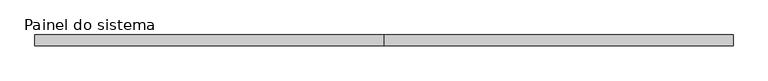
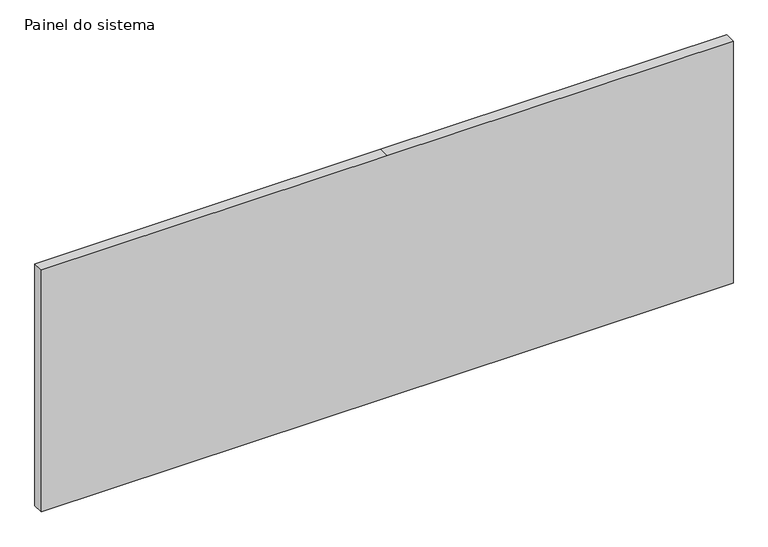
"""IFC4 building model written with IfcOpenShell, lengths in millimetres: plate geometry, Painel do sistema : Envidraçado."""

import ifcopenshell
import ifcopenshell.guid

model = None  # the IFC model being written
_history = None  # IfcOwnerHistory: only IFC2X3 demands one
_inside = {}  # id of a spatial element -> (the spatial element, [elements in it])
_under = {}  # id of a project, library or spatial element -> (it, [spatial elements below it])
_declared = {}  # id of a project -> (the project, [libraries it declares])
_typed = {}  # id of a type object -> (the type object, [elements of that type])
_made_of = {}  # id of a material, layer set ... -> (it, [elements and type objects made of it])


def new_model(schema):
    """Start an empty IFC model of exactly this schema.

    Asked for "IFC4X3", IfcOpenShell would pick the latest addendum, in which some entities
    have other attributes; the version numbers below select the first issue.
    IFC2X3 requires an IfcOwnerHistory on every rooted entity: one is made here for all.
    """
    global model, _history
    if schema == "IFC4X3":
        model = ifcopenshell.file(schema_version=(4, 3, 0, 0))
    else:
        model = ifcopenshell.file(schema=schema)
    _inside.clear()
    _under.clear()
    _declared.clear()
    _typed.clear()
    _made_of.clear()
    _history = None
    if model.schema == "IFC2X3":
        org = make("IfcOrganization", Name="unknown")
        user = make(
            "IfcPersonAndOrganization",
            ThePerson=make("IfcPerson", FamilyName="unknown"),
            TheOrganization=org,
        )
        app = make(
            "IfcApplication",
            ApplicationDeveloper=org,
            Version="unknown",
            ApplicationFullName="unknown",
            ApplicationIdentifier="unknown",
        )
        _history = make(
            "IfcOwnerHistory",
            OwningUser=user,
            OwningApplication=app,
            ChangeAction="ADDED",
            CreationDate=0,
        )
    return model


def make(cls, **values):
    """One entity of the class cls with the attributes given. An attribute that is None is left unset."""
    return model.create_entity(
        cls, **{name: value for name, value in values.items() if value is not None}
    )


def rooted(cls, **values):
    """An entity with a GlobalId (a new one), such as an element, a storey or a relation."""
    return make(cls, GlobalId=ifcopenshell.guid.new(), OwnerHistory=_history, **values)


def si_unit(unit_type, name, prefix=None):
    """IfcSIUnit, for example si_unit("LENGTHUNIT", "METRE", prefix="MILLI")."""
    return make("IfcSIUnit", UnitType=unit_type, Prefix=prefix, Name=name)


def assignment(units):
    """IfcUnitAssignment: the units of a project."""
    return None if units is None else make("IfcUnitAssignment", Units=units)


def point(xyz):
    """IfcCartesianPoint."""
    return None if xyz is None else make("IfcCartesianPoint", Coordinates=xyz)


def direction(xyz):
    """IfcDirection."""
    return None if xyz is None else make("IfcDirection", DirectionRatios=xyz)


def frame(location, z_axis=None, x_axis=None):
    """IfcAxis2Placement3D, a coordinate frame: its origin and axes. An axis left out is left unset."""
    return make(
        "IfcAxis2Placement3D",
        Location=point(location),
        Axis=direction(z_axis),
        RefDirection=direction(x_axis),
    )


def origin():
    """The frame at (0, 0, 0) with its axes left unset."""
    return frame((0.0, 0.0, 0.0))


def place(relative_to, where):
    """IfcLocalPlacement: puts the frame where relative to a parent placement (None: the world)."""
    return make(
        "IfcLocalPlacement", PlacementRelTo=relative_to, RelativePlacement=where
    )


def context(
    kind, dimensions, precision=None, world=None, true_north=None, identifier=None
):
    """IfcGeometricRepresentationContext, for example the 3D "Model" context."""
    return make(
        "IfcGeometricRepresentationContext",
        ContextIdentifier=identifier,
        ContextType=kind,
        CoordinateSpaceDimension=dimensions,
        Precision=precision,
        WorldCoordinateSystem=world,
        TrueNorth=true_north,
    )


def project(units=None, contexts=None):
    """IfcProject with its units and contexts."""
    return rooted(
        "IfcProject",
        Name="project",
        RepresentationContexts=contexts,
        UnitsInContext=assignment(units),
    )


def spatial(cls, under=None, at=None, **own):
    """A site, building, storey or space (cls), placed at a placement, below another one or the project."""
    s = rooted(cls, ObjectPlacement=at, **own)
    if under is not None:
        _under.setdefault(under.id(), (under, []))[1].append(s)
    return s


def polyline(points):
    """IfcPolyline through the points."""
    return make("IfcPolyline", Points=[point(p) for p in points])


def outline(outer, holes=None, kind="AREA"):
    """IfcArbitraryClosedProfileDef: a profile drawn as a closed curve; with holes, ...WithVoids."""
    if holes is None:
        return make("IfcArbitraryClosedProfileDef", ProfileType=kind, OuterCurve=outer)
    return make(
        "IfcArbitraryProfileDefWithVoids",
        ProfileType=kind,
        OuterCurve=outer,
        InnerCurves=holes,
    )


def extrude(swept, where, along, depth):
    """IfcExtrudedAreaSolid: the profile swept, set in the frame where, extruded along a direction by depth."""
    return make(
        "IfcExtrudedAreaSolid",
        SweptArea=swept,
        Position=where,
        ExtrudedDirection=direction(along),
        Depth=depth,
    )


def shape(context_of_items, identifier, shape_type, items):
    """IfcShapeRepresentation: the items that make up one representation, for example the "Body"."""
    return make(
        "IfcShapeRepresentation",
        ContextOfItems=context_of_items,
        RepresentationIdentifier=identifier,
        RepresentationType=shape_type,
        Items=items,
    )


def source(mapping_origin, context_of_items, identifier, shape_type, items):
    """IfcRepresentationMap: a shape defined once, which mapped items show again and again."""
    return make(
        "IfcRepresentationMap",
        MappingOrigin=mapping_origin,
        MappedRepresentation=shape(context_of_items, identifier, shape_type, items),
    )


def transform(
    local_origin,
    x_axis=None,
    y_axis=None,
    z_axis=None,
    scale=None,
    scale2=None,
    scale3=None,
    uniform=True,
):
    """IfcCartesianTransformationOperator3D, or its non-uniform kind. x_axis, y_axis, z_axis: its Axis1, 2, 3."""
    if uniform:
        return make(
            "IfcCartesianTransformationOperator3D",
            Axis1=direction(x_axis),
            Axis2=direction(y_axis),
            LocalOrigin=point(local_origin),
            Scale=scale,
            Axis3=direction(z_axis),
        )
    return make(
        "IfcCartesianTransformationOperator3DnonUniform",
        Axis1=direction(x_axis),
        Axis2=direction(y_axis),
        LocalOrigin=point(local_origin),
        Scale=scale,
        Axis3=direction(z_axis),
        Scale2=scale2,
        Scale3=scale3,
    )


def mapped(mapping_source, mapping_target):
    """IfcMappedItem: shows the shape of a source again, moved by a transform."""
    return make(
        "IfcMappedItem", MappingSource=mapping_source, MappingTarget=mapping_target
    )


def made_of(thing, what):
    """Note that an element or type object is made of a material, layer set ...; save() writes the relation."""
    if what is not None:
        _made_of.setdefault(what.id(), (what, []))[1].append(thing)
    return thing


def element(
    cls,
    number,
    at=None,
    inside=None,
    cuts=None,
    type_object=None,
    material=None,
    context=None,
    identifier="Body",
    shape_type=None,
    held_by="IfcProductDefinitionShape",
    body=None,
    shapes=None,
    **own,
):
    """One element of the class cls, such as IfcWall. Its Tag is "e" and its number.

    at: its placement. inside: the storey or other place that contains it. cuts: it is an
    opening in that element (IfcRelVoidsElement). A single representation is given by context,
    identifier, shape_type and body (its items); several are given by shapes. held_by: the class
    of the entity that holds the representations. save() writes the other relations.
    """
    e = rooted(cls, Tag="e%d" % number, ObjectPlacement=at, **own)
    if body is not None:
        shapes = [shape(context, identifier, shape_type, body)]
    if shapes is not None:
        e.Representation = make(held_by, Representations=shapes)
    if inside is not None:
        _inside.setdefault(inside.id(), (inside, []))[1].append(e)
    if cuts is not None:
        rooted(
            "IfcRelVoidsElement", RelatingBuildingElement=cuts, RelatedOpeningElement=e
        )
    if type_object is not None:
        _typed.setdefault(type_object.id(), (type_object, []))[1].append(e)
    return made_of(e, material)


def aggregate(whole, parts):
    """IfcRelAggregates: a whole, such as a stair, and the parts it consists of."""
    return rooted("IfcRelAggregates", RelatingObject=whole, RelatedObjects=parts)


def save(model, path):
    """Write the relations noted so far, then the file.

    IfcRelAggregates (storeys below a building ...), IfcRelContainedInSpatialStructure (elements
    in a storey), IfcRelDefinesByType, IfcRelAssociatesMaterial and IfcRelDeclares: one each for
    every whole, place, type object, material and project.
    """
    for whole, parts in _under.values():
        aggregate(whole, parts)
    for where, things in _inside.values():
        rooted(
            "IfcRelContainedInSpatialStructure",
            RelatedElements=things,
            RelatingStructure=where,
        )
    for kind, things in _typed.values():
        rooted("IfcRelDefinesByType", RelatedObjects=things, RelatingType=kind)
    for what, things in _made_of.values():
        rooted("IfcRelAssociatesMaterial", RelatedObjects=things, RelatingMaterial=what)
    for by, libraries in _declared.values():
        rooted("IfcRelDeclares", RelatingContext=by, RelatedDefinitions=libraries)
    model.write(path)


def painel_do_sistema_93f97b9b(model_context):
    return source(origin(), model_context, "Body", "SweptSolid", [
        extrude(outline(polyline([(0.0, -797.8166666), (0.0, 0.0), (0.0, 797.8166666), (590.0, 797.8166666), (590.0, 0.0), (590.0, -797.8166666), (0.0, -797.8166666)])), frame((0.0, -49.5, 0.0), z_axis=(0.0, 1.0, 0.0), x_axis=(0.0, 0.0, 1.0)), (0.0, 0.0, 1.0), 25.0),
    ])


if __name__ == "__main__":
    model = new_model("IFC4")
    model_context = context("Model", 3, world=origin())
    ifc_project = project(units=[si_unit("LENGTHUNIT", "METRE", prefix="MILLI")], contexts=[model_context])
    site = spatial("IfcSite", under=ifc_project)
    building = spatial("IfcBuilding", under=site)
    placement = place(None, origin())
    painel_do_sistema_shape = painel_do_sistema_93f97b9b(model_context)
    element("IfcPlate", 1, ObjectType="Painel do sistema : Envidraçado", at=placement, inside=building, context=model_context, shape_type="MappedRepresentation", body=[
        mapped(painel_do_sistema_shape, transform((0.0, 0.0, 0.0), x_axis=(1.0, 0.0, 0.0), y_axis=(0.0, 1.0, 0.0), z_axis=(0.0, 0.0, 1.0))),
    ])
    save(model, "model.ifc")

# Revit data of these elements
# Type "Painel do sistema : Envidraçado"
#   Construction Type Id = "GSP4R"
#   Analytic Construction = "Vidraça única Pilkington 1/8 pol"
#   Visual Light Transmittance = 0.9
#   Solar Heat Gain Coefficient = 0.86
#   Heat Transfer Coefficient (U) = 6.7069 W/(m²·K)
# Element 1 (IfcPlate, "Painel do sistema : Envidraçado")
#   Materials on its faces: ".VIDRO GENÉRICO"
# Materials
#   ".VIDRO GENÉRICO": class ".CC_VIDRO", colour RGB 0 128 192, transparency 0.9, Description = "Vidro comum", Cost = 0
